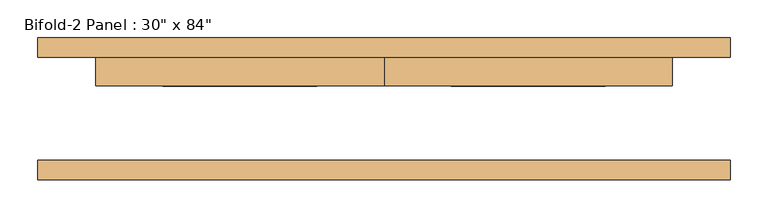
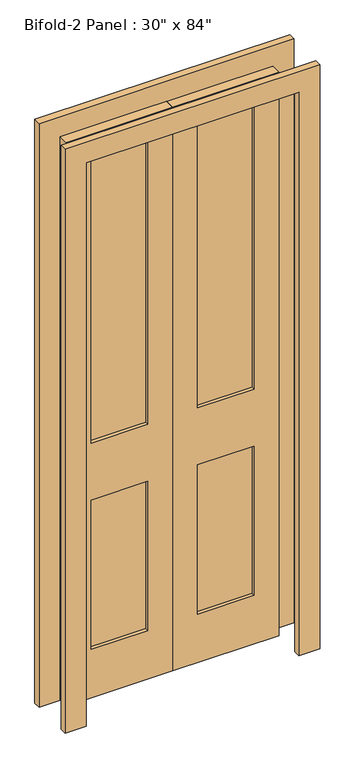
"""IFC4 building model written with IfcOpenShell, lengths in millimetres: door geometry."""

from ifc_helpers import new_model, si_unit, frame, origin, place, context, project, spatial, polyline, outline, extrude, source, transform, mapped, element, save


def door_bb229190(model_context):
    return source(origin(), model_context, "Body", "SweptSolid", [
        extrude(outline(polyline([(2133.6, 0.0), (2133.6, -381.0), (0.0, -381.0), (0.0, 0.0), (2133.6, 0.0)]), holes=[polyline([(2044.7, -88.9), (965.11872, -88.9), (965.11872, -292.1), (2044.7, -292.1), (2044.7, -88.9)]), polyline([(749.3, -88.9), (184.15, -88.9), (184.15, -292.1), (749.3, -292.1), (749.3, -88.9)])]), frame((0.0, 30.1625, 0.0), z_axis=(0.0, 1.0, 0.0), x_axis=(0.0, 0.0, 1.0)), (0.0, 0.0, 1.0), 38.1),
        extrude(outline(polyline([(-88.9, 42.8625), (-292.1, 42.8625), (-292.1, 55.5625), (-88.9, 55.5625), (-88.9, 42.8625)])), frame((0.0, 0.0, 965.11872), z_axis=(0.0, 0.0, 1.0), x_axis=(1.0, 0.0, 0.0)), (0.0, 0.0, 1.0), 1079.58128),
        extrude(outline(polyline([(-88.9, 42.8625), (-292.1, 42.8625), (-292.1, 55.5625), (-88.9, 55.5625), (-88.9, 42.8625)])), frame((0.0, 0.0, 184.15), z_axis=(0.0, 0.0, 1.0), x_axis=(1.0, 0.0, 0.0)), (0.0, 0.0, 1.0), 565.15),
        extrude(outline(polyline([(292.1, 42.8625), (88.9, 42.8625), (88.9, 55.5625), (292.1, 55.5625), (292.1, 42.8625)])), frame((0.0, 0.0, 965.11872), z_axis=(0.0, 0.0, 1.0), x_axis=(1.0, 0.0, 0.0)), (0.0, 0.0, 1.0), 1079.58128),
        extrude(outline(polyline([(292.1, 42.8625), (88.9, 42.8625), (88.9, 55.5625), (292.1, 55.5625), (292.1, 42.8625)])), frame((0.0, 0.0, 184.15), z_axis=(0.0, 0.0, 1.0), x_axis=(1.0, 0.0, 0.0)), (0.0, 0.0, 1.0), 565.15),
        extrude(outline(polyline([(2209.8, -457.2), (0.0, -457.2), (0.0, -381.0), (2133.6, -381.0), (2133.6, 381.0), (0.0, 381.0), (0.0, 457.2), (2209.8, 457.2), (2209.8, -457.2)])), frame((0.0, 68.2625, 0.0), z_axis=(0.0, 1.0, 0.0), x_axis=(0.0, 0.0, 1.0)), (0.0, 0.0, 1.0), 25.4),
        extrude(outline(polyline([(2209.8, 457.2), (2209.8, -457.2), (0.0, -457.2), (0.0, -381.0), (2133.6, -381.0), (2133.6, 381.0), (0.0, 381.0), (0.0, 457.2), (2209.8, 457.2)])), frame((0.0, -93.6625, 0.0), z_axis=(0.0, 1.0, 0.0), x_axis=(0.0, 0.0, 1.0)), (0.0, 0.0, 1.0), 25.4),
        extrude(outline(polyline([(2133.6, 381.0), (2133.6, 0.0), (0.0, 0.0), (0.0, 381.0), (2133.6, 381.0)]), holes=[polyline([(2044.7, 88.9), (2044.7, 292.1), (965.11872, 292.1), (965.11872, 88.9), (2044.7, 88.9)]), polyline([(749.3, 88.9), (749.3, 292.1), (184.15, 292.1), (184.15, 88.9), (749.3, 88.9)])]), frame((0.0, 30.1625, 0.0), z_axis=(0.0, 1.0, 0.0), x_axis=(0.0, 0.0, 1.0)), (0.0, 0.0, 1.0), 38.1),
    ])


if __name__ == "__main__":
    model = new_model("IFC4")
    model_context = context("Model", 3, world=origin())
    ifc_project = project(units=[si_unit("LENGTHUNIT", "METRE", prefix="MILLI")], contexts=[model_context])
    site = spatial("IfcSite", under=ifc_project)
    building = spatial("IfcBuilding", under=site)
    placement = place(None, origin())
    door_shape = door_bb229190(model_context)
    element("IfcDoor", 1, ObjectType="Bifold-2 Panel : 30\" x 84\"", at=placement, inside=building, context=model_context, shape_type="MappedRepresentation", body=[
        mapped(door_shape, transform((0.0, 0.0, 0.0), x_axis=(1.0, 0.0, 0.0), y_axis=(0.0, 1.0, 0.0), z_axis=(0.0, 0.0, 1.0))),
    ])
    save(model, "model.ifc")

# Revit data of these elements
# Type "Bifold-2 Panel : 30\" x 84\""
#   Type Mark = "35"
#   Assembly Code = "C1020"
#   Thickness = 0' - 1 1/2"
#   Height = 7' - 0"
#   Trim Projection Ext = 0' - 1"
#   Trim Projection Int = 0' - 1"
#   Trim Width = 0' - 3"
#   Width = 2' - 6"
#   Door Material = Door - Panel
#   Frame Material = Door - Frame
#   Function = (empty or 0)
#   Wall Closure = (empty or 0)
# Element 1 (IfcDoor, "Bifold-2 Panel : 30\" x 84\"")
#   Materials on its faces: "Door - Panel", "Door - Frame"
# Materials
#   "Door - Panel": class "Wood", colour RGB 210 159 95, transparency 0, Cost = 0
#   "Door - Frame": class "Miscellaneous", colour RGB 118 70 51, transparency 0, Cost = 0
